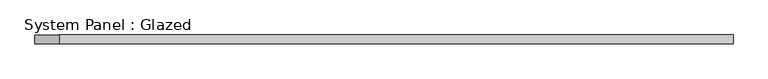
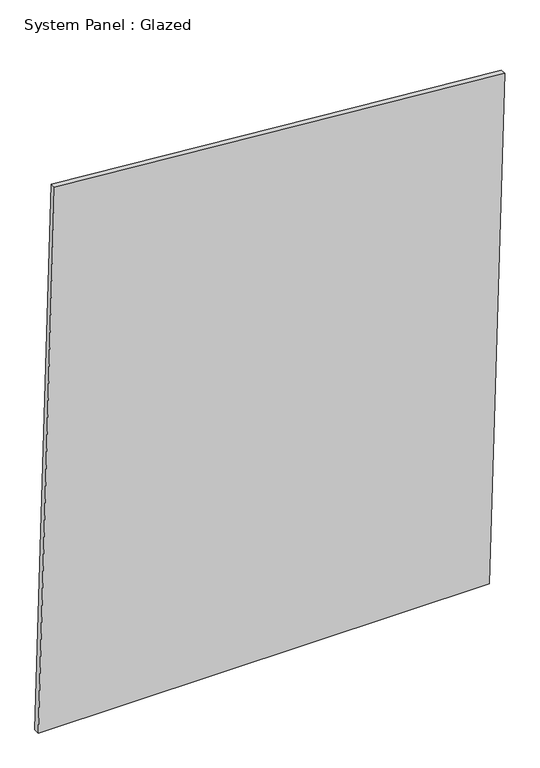
"""IFC4 building model written with IfcOpenShell, lengths in millimetres: plate geometry, System Panel : Glazed."""

from ifc_helpers import new_model, si_unit, frame, origin, place, context, project, spatial, polyline, outline, extrude, source, transform, mapped, element, save


def system_panel_glazed_c41e03b4(model_context):
    return source(origin(), model_context, "Body", "SweptSolid", [
        extrude(outline(polyline([(0.0, -1008.7560992), (0.0, 941.2557286), (2310.4175162, 1008.7560992), (2471.2238346, -938.6456704), (0.0, -1008.7560992)])), frame((0.0, -49.5, 0.0), z_axis=(0.0, 1.0, 0.0), x_axis=(0.0, 0.0, 1.0)), (0.0, 0.0, 1.0), 25.0),
    ])


if __name__ == "__main__":
    model = new_model("IFC4")
    model_context = context("Model", 3, world=origin())
    ifc_project = project(units=[si_unit("LENGTHUNIT", "METRE", prefix="MILLI")], contexts=[model_context])
    site = spatial("IfcSite", under=ifc_project)
    building = spatial("IfcBuilding", under=site)
    placement = place(None, origin())
    system_panel_glazed_shape = system_panel_glazed_c41e03b4(model_context)
    element("IfcPlate", 1, ObjectType="System Panel : Glazed", at=placement, inside=building, context=model_context, shape_type="MappedRepresentation", body=[
        mapped(system_panel_glazed_shape, transform((0.0, 0.0, 0.0), x_axis=(1.0, 0.0, 0.0), y_axis=(0.0, 1.0, 0.0), z_axis=(0.0, 0.0, 1.0))),
    ])
    save(model, "model.ifc")

# Revit data of these elements
# Element 1 (IfcPlate, "System Panel : Glazed")
#   Materials on its faces: "Glass, Clear Glazing"
# Materials
#   "Glass, Clear Glazing": class "Glass", colour RGB 247 249 248, transparency 0.85, Description = "Clear glazing", Cost = 0
